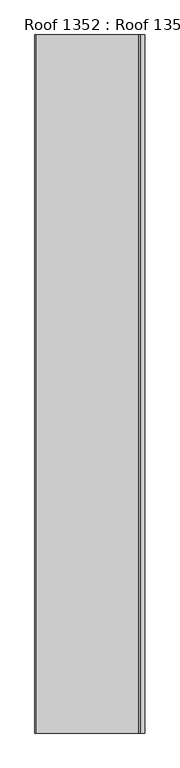
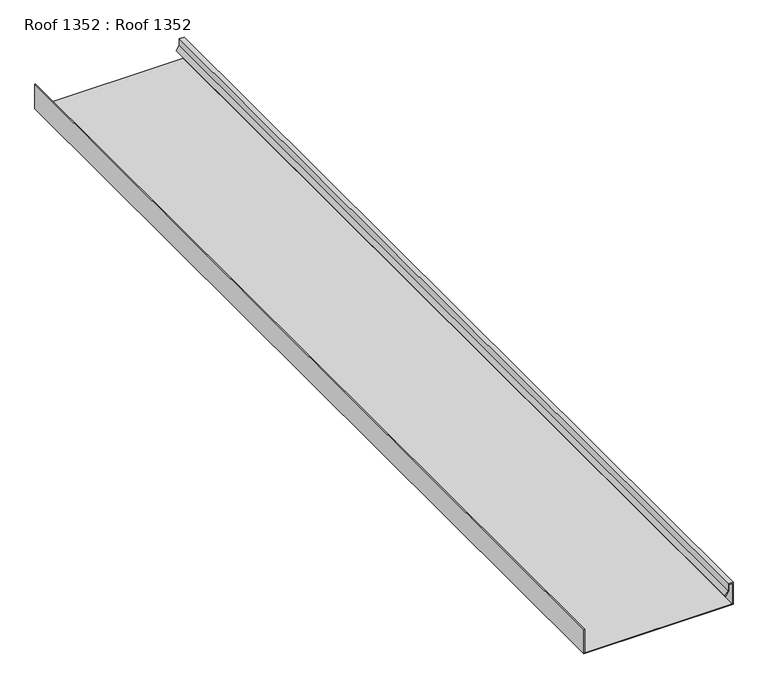
"""IFC4 building model written with IfcOpenShell, lengths in millimetres: proxy geometry, Roof 1352 : Roof 1352."""

from ifc_helpers import new_model, si_unit, frame, origin, place, context, project, spatial, polyline, outline, extrude, source, transform, mapped, element, save


def roof_1352_roof_1352_30324008(model_context):
    return source(origin(), model_context, "Body", "SweptSolid", [
        extrude(outline(polyline([(43489.1054687, -6143.2617188), (43502.590625, -6143.2617188), (43502.590625, -6136.5869141), (43457.7734375, -6136.5869141), (43457.7734375, -6447.0209961), (43509.546875, -6447.0209961), (43509.546875, -6449.0209961), (43455.7734375, -6449.0209961), (43455.7734375, -6134.5869141), (43504.590625, -6134.5869141), (43504.590625, -6145.2617187), (43489.754523, -6145.2617187), (43480.4712961, -6151.9963099), (43479.296875, -6150.3774414), (43489.1054687, -6143.2617188)])), frame((0.0, 7982.1531721, 0.0), z_axis=(0.0, 1.0, 0.0), x_axis=(0.0, 0.0, 1.0)), (0.0, 0.0, 1.0), 2000.0),
    ])


if __name__ == "__main__":
    model = new_model("IFC4")
    model_context = context("Model", 3, world=origin())
    ifc_project = project(units=[si_unit("LENGTHUNIT", "METRE", prefix="MILLI")], contexts=[model_context])
    site = spatial("IfcSite", under=ifc_project)
    building = spatial("IfcBuilding", under=site)
    placement = place(None, origin())
    roof_1352_roof_1352_shape = roof_1352_roof_1352_30324008(model_context)
    element("IfcBuildingElementProxy", 1, Name="Roof 1352 : Roof 1352", ObjectType="Roof 1352 : Roof 1352", at=placement, inside=building, context=model_context, shape_type="MappedRepresentation", body=[
        mapped(roof_1352_roof_1352_shape, transform((0.0, 0.0, 0.0), x_axis=(1.0, 0.0, 0.0), y_axis=(0.0, 1.0, 0.0), z_axis=(0.0, 0.0, 1.0))),
    ])
    save(model, "model.ifc")

# Revit data of these elements
# Type "Roof 1352 : Roof 1352"
#   NameOverride = "Roof"
# Element 1 (IfcBuildingElementProxy, "Roof 1352 : Roof 1352")
#   Materials on its faces: "STANDING SEAM METAL ROOF FOLLOW MANU. RECOMMENDED EDGE/TRANSITION DETAILS"
# Materials
#   "STANDING SEAM METAL ROOF FOLLOW MANU. RECOMMENDED EDGE/TRANSITION DETAILS": class "Unassigned", colour RGB 128 128 128, transparency 0, Cost = 0
